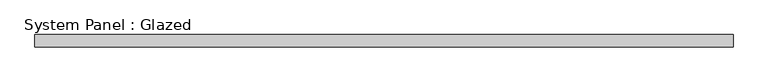
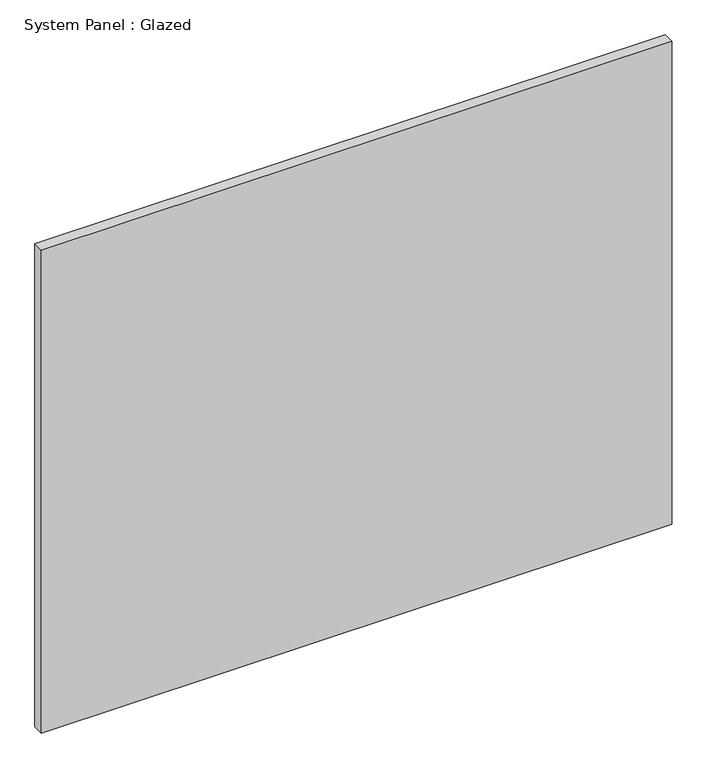
"""IFC4 building model written with IfcOpenShell, lengths in millimetres: plate geometry, System Panel : Glazed."""

from ifc_helpers import new_model, si_unit, origin, origin_with_axes, place, context, project, spatial, polyline, outline, extrude, source, transform, mapped, element, save


def system_panel_glazed_8e8b8cb0(model_context):
    return source(origin(), model_context, "Body", "SweptSolid", [
        extrude(outline(polyline([(713.3166666, 19.05), (-713.3166666, 19.05), (-713.3166666, 44.45), (713.3166666, 44.45), (713.3166666, 19.05)])), origin_with_axes(), (0.0, 0.0, 1.0), 1155.7),
    ])


if __name__ == "__main__":
    model = new_model("IFC4")
    model_context = context("Model", 3, world=origin())
    ifc_project = project(units=[si_unit("LENGTHUNIT", "METRE", prefix="MILLI")], contexts=[model_context])
    site = spatial("IfcSite", under=ifc_project)
    building = spatial("IfcBuilding", under=site)
    placement = place(None, origin())
    system_panel_glazed_shape = system_panel_glazed_8e8b8cb0(model_context)
    element("IfcPlate", 1, ObjectType="System Panel : Glazed", at=placement, inside=building, context=model_context, shape_type="MappedRepresentation", body=[
        mapped(system_panel_glazed_shape, transform((0.0, 0.0, 0.0), x_axis=(1.0, 0.0, 0.0), y_axis=(0.0, 1.0, 0.0), z_axis=(0.0, 0.0, 1.0))),
    ])
    save(model, "model.ifc")

# Revit data of these elements
# Type "System Panel : Glazed"
#   Construction Type Id = "GSP4R"
#   Analytic Construction = "1/8 in Pilkington single glazing"
#   Visual Light Transmittance = 0.9
#   Solar Heat Gain Coefficient = 0.86
#   Heat Transfer Coefficient (U) = 1.18115 BTU/(h·ft²·°F)
#   Define Thermal Properties by = 1
# Element 1 (IfcPlate, "System Panel : Glazed")
#   Materials on its faces: "Glass"
# Materials
#   "Glass": class "Glass", colour RGB 0 128 192, transparency 0.75, Description = "Soda Lime Glass", Cost = 0
